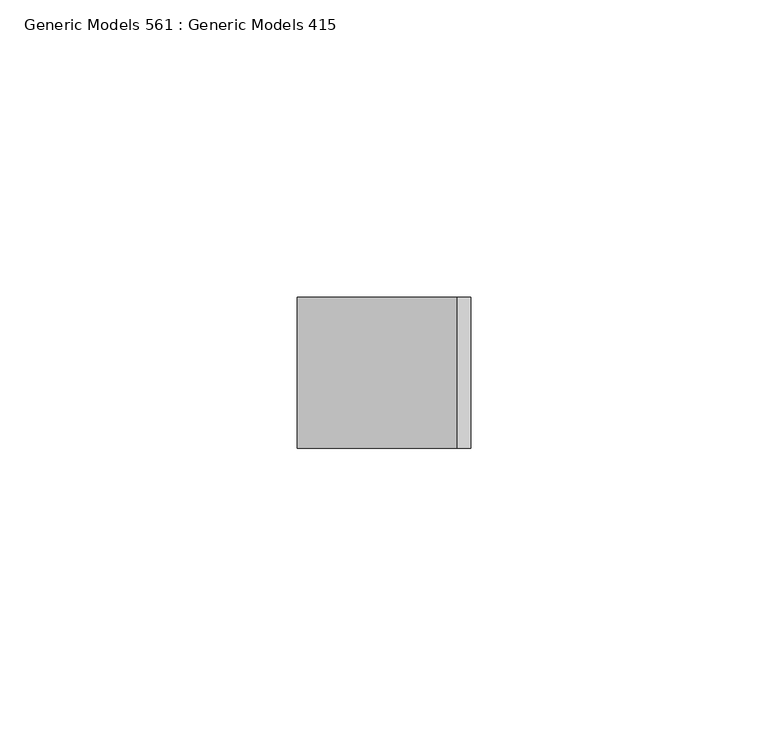
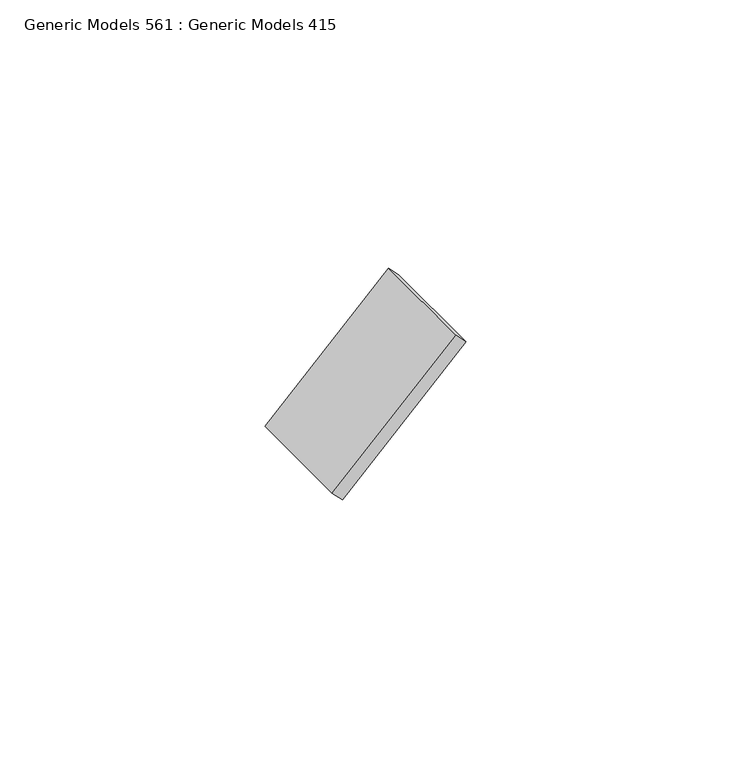
"""IFC4 building model written with IfcOpenShell, lengths in millimetres: proxy geometry, Generic Models 561 : Generic Models 415."""

import ifcopenshell
import ifcopenshell.guid

model = None  # the IFC model being written
_history = None  # IfcOwnerHistory: only IFC2X3 demands one
_inside = {}  # id of a spatial element -> (the spatial element, [elements in it])
_under = {}  # id of a project, library or spatial element -> (it, [spatial elements below it])
_declared = {}  # id of a project -> (the project, [libraries it declares])
_typed = {}  # id of a type object -> (the type object, [elements of that type])
_made_of = {}  # id of a material, layer set ... -> (it, [elements and type objects made of it])


def new_model(schema):
    """Start an empty IFC model of exactly this schema.

    Asked for "IFC4X3", IfcOpenShell would pick the latest addendum, in which some entities
    have other attributes; the version numbers below select the first issue.
    IFC2X3 requires an IfcOwnerHistory on every rooted entity: one is made here for all.
    """
    global model, _history
    if schema == "IFC4X3":
        model = ifcopenshell.file(schema_version=(4, 3, 0, 0))
    else:
        model = ifcopenshell.file(schema=schema)
    _inside.clear()
    _under.clear()
    _declared.clear()
    _typed.clear()
    _made_of.clear()
    _history = None
    if model.schema == "IFC2X3":
        org = make("IfcOrganization", Name="unknown")
        user = make(
            "IfcPersonAndOrganization",
            ThePerson=make("IfcPerson", FamilyName="unknown"),
            TheOrganization=org,
        )
        app = make(
            "IfcApplication",
            ApplicationDeveloper=org,
            Version="unknown",
            ApplicationFullName="unknown",
            ApplicationIdentifier="unknown",
        )
        _history = make(
            "IfcOwnerHistory",
            OwningUser=user,
            OwningApplication=app,
            ChangeAction="ADDED",
            CreationDate=0,
        )
    return model


def make(cls, **values):
    """One entity of the class cls with the attributes given. An attribute that is None is left unset."""
    return model.create_entity(
        cls, **{name: value for name, value in values.items() if value is not None}
    )


def rooted(cls, **values):
    """An entity with a GlobalId (a new one), such as an element, a storey or a relation."""
    return make(cls, GlobalId=ifcopenshell.guid.new(), OwnerHistory=_history, **values)


def si_unit(unit_type, name, prefix=None):
    """IfcSIUnit, for example si_unit("LENGTHUNIT", "METRE", prefix="MILLI")."""
    return make("IfcSIUnit", UnitType=unit_type, Prefix=prefix, Name=name)


def assignment(units):
    """IfcUnitAssignment: the units of a project."""
    return None if units is None else make("IfcUnitAssignment", Units=units)


def point(xyz):
    """IfcCartesianPoint."""
    return None if xyz is None else make("IfcCartesianPoint", Coordinates=xyz)


def direction(xyz):
    """IfcDirection."""
    return None if xyz is None else make("IfcDirection", DirectionRatios=xyz)


def frame(location, z_axis=None, x_axis=None):
    """IfcAxis2Placement3D, a coordinate frame: its origin and axes. An axis left out is left unset."""
    return make(
        "IfcAxis2Placement3D",
        Location=point(location),
        Axis=direction(z_axis),
        RefDirection=direction(x_axis),
    )


def origin():
    """The frame at (0, 0, 0) with its axes left unset."""
    return frame((0.0, 0.0, 0.0))


def place(relative_to, where):
    """IfcLocalPlacement: puts the frame where relative to a parent placement (None: the world)."""
    return make(
        "IfcLocalPlacement", PlacementRelTo=relative_to, RelativePlacement=where
    )


def context(
    kind, dimensions, precision=None, world=None, true_north=None, identifier=None
):
    """IfcGeometricRepresentationContext, for example the 3D "Model" context."""
    return make(
        "IfcGeometricRepresentationContext",
        ContextIdentifier=identifier,
        ContextType=kind,
        CoordinateSpaceDimension=dimensions,
        Precision=precision,
        WorldCoordinateSystem=world,
        TrueNorth=true_north,
    )


def project(units=None, contexts=None):
    """IfcProject with its units and contexts."""
    return rooted(
        "IfcProject",
        Name="project",
        RepresentationContexts=contexts,
        UnitsInContext=assignment(units),
    )


def spatial(cls, under=None, at=None, **own):
    """A site, building, storey or space (cls), placed at a placement, below another one or the project."""
    s = rooted(cls, ObjectPlacement=at, **own)
    if under is not None:
        _under.setdefault(under.id(), (under, []))[1].append(s)
    return s


def polyline(points):
    """IfcPolyline through the points."""
    return make("IfcPolyline", Points=[point(p) for p in points])


def outline(outer, holes=None, kind="AREA"):
    """IfcArbitraryClosedProfileDef: a profile drawn as a closed curve; with holes, ...WithVoids."""
    if holes is None:
        return make("IfcArbitraryClosedProfileDef", ProfileType=kind, OuterCurve=outer)
    return make(
        "IfcArbitraryProfileDefWithVoids",
        ProfileType=kind,
        OuterCurve=outer,
        InnerCurves=holes,
    )


def extrude(swept, where, along, depth):
    """IfcExtrudedAreaSolid: the profile swept, set in the frame where, extruded along a direction by depth."""
    return make(
        "IfcExtrudedAreaSolid",
        SweptArea=swept,
        Position=where,
        ExtrudedDirection=direction(along),
        Depth=depth,
    )


def shape(context_of_items, identifier, shape_type, items):
    """IfcShapeRepresentation: the items that make up one representation, for example the "Body"."""
    return make(
        "IfcShapeRepresentation",
        ContextOfItems=context_of_items,
        RepresentationIdentifier=identifier,
        RepresentationType=shape_type,
        Items=items,
    )


def source(mapping_origin, context_of_items, identifier, shape_type, items):
    """IfcRepresentationMap: a shape defined once, which mapped items show again and again."""
    return make(
        "IfcRepresentationMap",
        MappingOrigin=mapping_origin,
        MappedRepresentation=shape(context_of_items, identifier, shape_type, items),
    )


def transform(
    local_origin,
    x_axis=None,
    y_axis=None,
    z_axis=None,
    scale=None,
    scale2=None,
    scale3=None,
    uniform=True,
):
    """IfcCartesianTransformationOperator3D, or its non-uniform kind. x_axis, y_axis, z_axis: its Axis1, 2, 3."""
    if uniform:
        return make(
            "IfcCartesianTransformationOperator3D",
            Axis1=direction(x_axis),
            Axis2=direction(y_axis),
            LocalOrigin=point(local_origin),
            Scale=scale,
            Axis3=direction(z_axis),
        )
    return make(
        "IfcCartesianTransformationOperator3DnonUniform",
        Axis1=direction(x_axis),
        Axis2=direction(y_axis),
        LocalOrigin=point(local_origin),
        Scale=scale,
        Axis3=direction(z_axis),
        Scale2=scale2,
        Scale3=scale3,
    )


def mapped(mapping_source, mapping_target):
    """IfcMappedItem: shows the shape of a source again, moved by a transform."""
    return make(
        "IfcMappedItem", MappingSource=mapping_source, MappingTarget=mapping_target
    )


def made_of(thing, what):
    """Note that an element or type object is made of a material, layer set ...; save() writes the relation."""
    if what is not None:
        _made_of.setdefault(what.id(), (what, []))[1].append(thing)
    return thing


def element(
    cls,
    number,
    at=None,
    inside=None,
    cuts=None,
    type_object=None,
    material=None,
    context=None,
    identifier="Body",
    shape_type=None,
    held_by="IfcProductDefinitionShape",
    body=None,
    shapes=None,
    **own,
):
    """One element of the class cls, such as IfcWall. Its Tag is "e" and its number.

    at: its placement. inside: the storey or other place that contains it. cuts: it is an
    opening in that element (IfcRelVoidsElement). A single representation is given by context,
    identifier, shape_type and body (its items); several are given by shapes. held_by: the class
    of the entity that holds the representations. save() writes the other relations.
    """
    e = rooted(cls, Tag="e%d" % number, ObjectPlacement=at, **own)
    if body is not None:
        shapes = [shape(context, identifier, shape_type, body)]
    if shapes is not None:
        e.Representation = make(held_by, Representations=shapes)
    if inside is not None:
        _inside.setdefault(inside.id(), (inside, []))[1].append(e)
    if cuts is not None:
        rooted(
            "IfcRelVoidsElement", RelatingBuildingElement=cuts, RelatedOpeningElement=e
        )
    if type_object is not None:
        _typed.setdefault(type_object.id(), (type_object, []))[1].append(e)
    return made_of(e, material)


def aggregate(whole, parts):
    """IfcRelAggregates: a whole, such as a stair, and the parts it consists of."""
    return rooted("IfcRelAggregates", RelatingObject=whole, RelatedObjects=parts)


def save(model, path):
    """Write the relations noted so far, then the file.

    IfcRelAggregates (storeys below a building ...), IfcRelContainedInSpatialStructure (elements
    in a storey), IfcRelDefinesByType, IfcRelAssociatesMaterial and IfcRelDeclares: one each for
    every whole, place, type object, material and project.
    """
    for whole, parts in _under.values():
        aggregate(whole, parts)
    for where, things in _inside.values():
        rooted(
            "IfcRelContainedInSpatialStructure",
            RelatedElements=things,
            RelatingStructure=where,
        )
    for kind, things in _typed.values():
        rooted("IfcRelDefinesByType", RelatedObjects=things, RelatingType=kind)
    for what, things in _made_of.values():
        rooted("IfcRelAssociatesMaterial", RelatedObjects=things, RelatingMaterial=what)
    for by, libraries in _declared.values():
        rooted("IfcRelDeclares", RelatingContext=by, RelatedDefinitions=libraries)
    model.write(path)


def generic_models_561_generic_models_415_9297ded0(model_context):
    return source(origin(), model_context, "Body", "SweptSolid", [
        extrude(outline(polyline([(0.0, -3.175), (0.0, 0.0), (25.4, 0.0), (25.4, -3.175), (0.0, -3.175)])), frame((7848.0411784, 4501.3863946, 124368.8849742), z_axis=(0.7071067811867181, 0.0, 0.707106781186377), x_axis=(0.0, -1.0, 0.0)), (0.0, 0.0, 1.0), 38.1),
    ])


if __name__ == "__main__":
    model = new_model("IFC4")
    model_context = context("Model", 3, world=origin())
    ifc_project = project(units=[si_unit("LENGTHUNIT", "METRE", prefix="MILLI")], contexts=[model_context])
    site = spatial("IfcSite", under=ifc_project)
    building = spatial("IfcBuilding", under=site)
    placement = place(None, origin())
    generic_models_561_generic_models_415_shape = generic_models_561_generic_models_415_9297ded0(model_context)
    element("IfcBuildingElementProxy", 1, Name="Generic Models 561 : Generic Models 415", ObjectType="Generic Models 561 : Generic Models 415", at=placement, inside=building, context=model_context, shape_type="MappedRepresentation", body=[
        mapped(generic_models_561_generic_models_415_shape, transform((0.0, 0.0, 0.0), x_axis=(1.0, 0.0, 0.0), y_axis=(0.0, 1.0, 0.0), z_axis=(0.0, 0.0, 1.0))),
    ])
    save(model, "model.ifc")

# Revit data of these elements
# Element 1 (IfcBuildingElementProxy, "Generic Models 561 : Generic Models 415")
#   Materials on its faces: "_WELDED STEEL TABS FOR LOUVER ATTACHMENT"
# Materials
#   "_WELDED STEEL TABS FOR LOUVER ATTACHMENT": class "Metal", colour RGB 199 199 199, transparency 0, Description = "Structural steel 50ksi", Cost = 0
